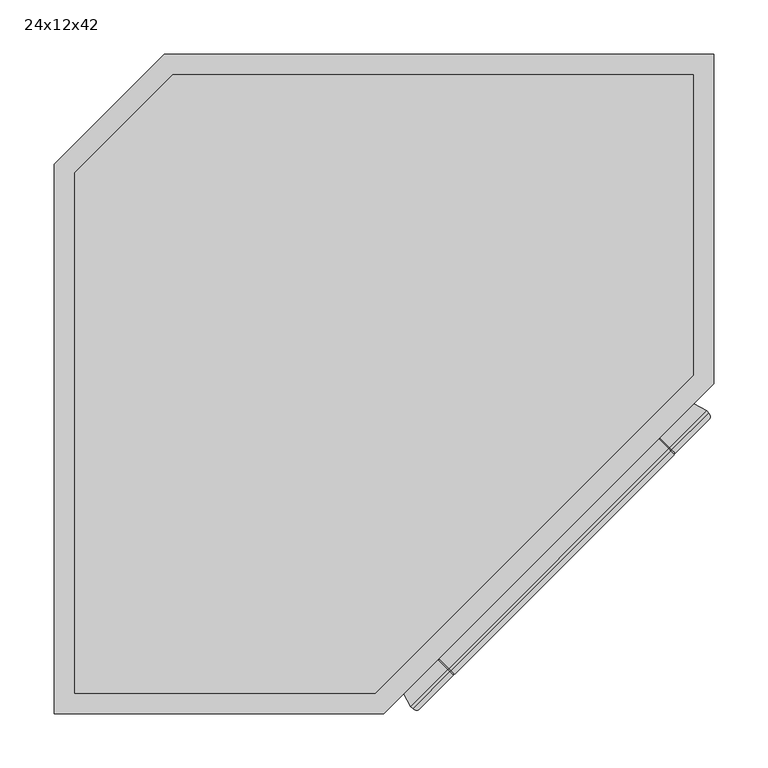
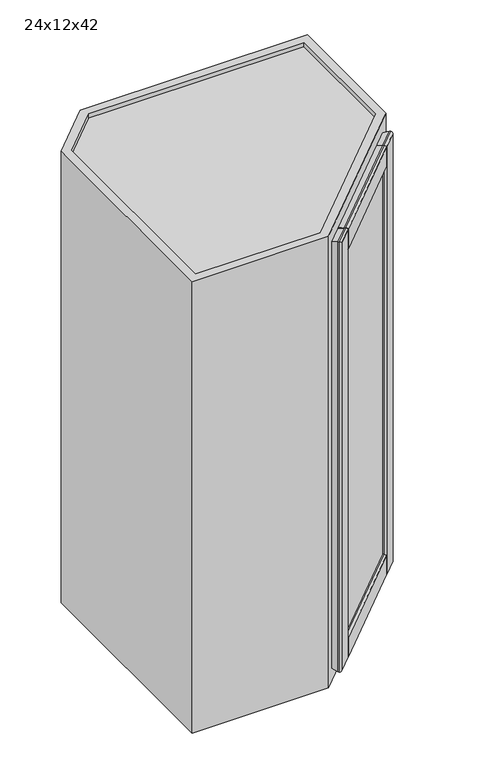
"""IFC4 building model written with IfcOpenShell, lengths in millimetres: furniture geometry, Cabinet-Wall-Merillat-Angle_Single_Door-Marlin : 24x12x42."""

from ifc_helpers import new_model, si_unit, frame, origin, place, context, project, spatial, polyline, circle_curve, ellipse_curve, outline, extrude, faceted_brep, source, transform, mapped, element, save
from ifc_brep_helpers import plane_surface, cylinder_surface, advanced_brep


def furniture_24x12x42_852458e2(model_context):
    return source(origin(), model_context, "Body", "SolidModel", [
        advanced_brep(
        [(-277.8609132, -57.3881325, 2451.1), (-277.8609132, -57.3881325, 1435.1), (-272.5103122, -58.3596318, 1438.1964925), (-272.5103122, -58.3596318, 2448.0035075), (-279.818609, -55.4304366, 2451.1), (-279.818609, -55.4304366, 1435.1), (-286.5897222, -43.7022222, 2447.5948), (-286.5897222, -43.7022222, 1438.6052), (-254.9849038, -12.0974038, 2402.8988372), (-254.1619151, -12.3969472, 2402.5287055), (-249.5344535, -14.0812055, 2400.4475465), (-249.5344535, -14.0812055, 1485.7524535), (-254.1619151, -12.3969472, 1483.6712945), (-254.9849038, -12.0974038, 1483.3011628), (-248.9402505, -16.6549814, 2401.847316), (-248.9402505, -16.6549814, 1484.352684), (-258.8946123, -26.9630247, 2416.175), (-258.8946123, -26.9630247, 1470.025), (-255.4821149, -30.3755221, 2416.175), (-255.4821149, -30.3755221, 1470.025), (-245.1740716, -20.4211603, 2401.847316), (-245.1740716, -20.4211603, 1484.352684), (-242.6002957, -21.0153633, 2400.4475465), (-242.6002957, -21.0153633, 1485.7524535), (-240.9160374, -25.6428249, 2402.5287055), (-240.6188146, -26.4594378, 2402.8959698), (-240.616494, -26.4658136, 1483.3011628), (-240.9160374, -25.6428249, 1483.6712945), (-3.5528682, 210.5978122, 1438.1964925), (-35.420563, 178.7301174, 1438.1964925), (-38.5816131, 181.8911676, 1435.1), (-4.5243675, 215.9484132, 1435.1), (-243.7755166, -23.3027358, 1435.1), (-240.6144664, -26.463786, 1438.1964925), (-242.6529845, -22.1802038, 1435.1), (-39.7041452, 180.7686356, 1435.1), (-36.543095, 177.6075854, 1438.1964925), (-239.4919344, -25.341254, 1438.1964925), (-40.539309, 183.8488634, 1435.1), (-6.4820634, 217.906109, 1435.1), (-245.7332124, -21.34504, 1435.1), (-244.6106804, -20.222508, 1435.1), (-41.661841, 182.7263314, 1435.1), (-49.7889728, 193.0985272, 1438.6052), (-18.2102778, 224.6772222, 1438.6052), (-254.9828762, -12.0953762, 1438.6052), (-253.8603442, -10.9728442, 1438.6052), (-50.9115048, 191.9759952, 1438.6052), (-47.8312945, 187.6219535, 1485.7524535), (-49.5155528, 192.2494151, 1483.6712945), (-50.3502388, 191.4147292, 1483.6712945), (-50.9115048, 191.9759952, 1483.3011628), (-253.8603442, -10.9728442, 1483.3011628), (-253.2990782, -11.5341102, 1483.6712945), (-45.2575186, 187.0277505, 1484.352684), (-34.9494753, 196.9821123, 1470.025), (-31.5369779, 193.5696149, 1470.025), (-41.4913397, 183.2615716, 1484.352684), (-40.8971367, 180.6877957, 1485.7524535), (-240.0532004, -24.779988, 1483.6712945), (-239.4919344, -25.341254, 1483.3011628), (-36.543095, 177.6075854, 1483.3011628), (-37.104361, 178.1688514, 1483.6712945), (-36.2696751, 179.0035374, 1483.6712945), (-4.5243675, 215.9484132, 2451.1), (-3.5528682, 210.5978122, 2448.0035075), (-6.4820634, 217.906109, 2451.1), (-18.2102778, 224.6772222, 2447.5948), (-49.8150962, 193.0724038, 1483.3011628), (-47.8312945, 187.6219535, 2400.4475465), (-49.5155528, 192.2494151, 2402.5287055), (-49.8150962, 193.0724038, 2402.8988372), (-45.2575186, 187.0277505, 2401.847316), (-34.9494753, 196.9821123, 2416.175), (-31.5369779, 193.5696149, 2416.175), (-41.4913397, 183.2615716, 2401.847316), (-40.8971367, 180.6877957, 2400.4475465), (-35.4466864, 178.703994, 1483.3011628), (-35.4466864, 178.703994, 2402.8988372), (-36.2696751, 179.0035374, 2402.5287055), (-240.6144664, -26.463786, 2448.0035075), (-243.7755166, -23.3027358, 2451.1), (-38.5816131, 181.8911676, 2451.1), (-35.420563, 178.7301174, 2448.0035075), (-39.7041452, 180.7686356, 2451.1), (-242.6529845, -22.1802038, 2451.1), (-239.4919344, -25.341254, 2448.0035075), (-36.543095, 177.6075854, 2448.0035075), (-245.7332124, -21.34504, 2451.1), (-40.539309, 183.8488634, 2451.1), (-41.661841, 182.7263314, 2451.1), (-244.6106804, -20.222508, 2451.1), (-254.9828762, -12.0953762, 2447.5948), (-49.7889728, 193.0985272, 2447.5948), (-50.9115048, 191.9759952, 2447.5948), (-253.8603442, -10.9728442, 2447.5948), (-50.9115048, 191.9759952, 2402.8988372), (-253.8603442, -10.9728442, 2402.8988372), (-253.2990782, -11.5341102, 2402.5287055), (-50.3502388, 191.4147292, 2402.5287055), (-37.104361, 178.1688514, 2402.5287055), (-36.543095, 177.6075854, 2402.8988372), (-239.4919344, -25.341254, 2402.8988372), (-240.0532004, -24.779988, 2402.5287055), (-37.104361, 178.1688514, 2447.8526052), (-39.7041452, 180.7686356, 2450.30625), (-41.5879457, 182.6524361, 2450.30625), (-50.3502388, 191.4147292, 2446.9857412), (-49.2277068, 192.5372612, 2402.5287055), (-49.2277068, 192.5372612, 2446.9857412), (-40.4654137, 183.7749682, 2450.30625), (-38.5816131, 181.8911676, 2450.30625), (-35.981829, 179.2913834, 2447.8526052), (-35.981829, 179.2913834, 2402.5287055), (-241.1757324, -25.90252, 2402.5287055), (-241.1757324, -25.90252, 2447.8526052), (-243.7755166, -23.3027358, 2450.30625), (-245.6593171, -21.4189353, 2450.30625), (-254.4216102, -12.6566422, 2446.9857412), (-254.4216102, -12.6566422, 2402.5287055), (-253.2990782, -11.5341102, 2446.9857412), (-244.5367851, -20.2964033, 2450.30625), (-242.6529845, -22.1802038, 2450.30625), (-240.0532004, -24.779988, 2447.8526052), (-254.4216102, -12.6566422, 1483.6712945), (-254.4216102, -12.6566422, 1439.2142588), (-245.6593171, -21.4189353, 1435.89375), (-243.7755166, -23.3027358, 1435.89375), (-241.1757324, -25.90252, 1438.3473948), (-241.1757324, -25.90252, 1483.6712945), (-240.0532004, -24.779988, 1438.3473948), (-242.6529845, -22.1802038, 1435.89375), (-244.5367851, -20.2964033, 1435.89375), (-253.2990782, -11.5341102, 1439.2142588), (-50.3502388, 191.4147292, 1439.2142588), (-41.5879457, 182.6524361, 1435.89375), (-39.7041452, 180.7686356, 1435.89375), (-37.104361, 178.1688514, 1438.3473948), (-35.981829, 179.2913834, 1483.6712945), (-35.981829, 179.2913834, 1438.3473948), (-38.5816131, 181.8911676, 1435.89375), (-40.4654137, 183.7749682, 1435.89375), (-49.2277068, 192.5372612, 1439.2142588), (-49.2277068, 192.5372612, 1483.6712945)],
        [
            (0, 1),
            (1, 2, ellipse_curve(frame((-274.4843369, -54.0115562, 1439.8752), z_axis=(-0.5000000000000054, -0.4999999999999945, 0.7071067811865475), x_axis=(0.5000000000000053, 0.4999999999999944, 0.7071067811865476)), 6.7531526, 4.7752)),
            (2, 3),
            (3, 0, ellipse_curve(frame((-274.4843369, -54.0115562, 2446.3248), z_axis=(-0.5000000000000054, -0.4999999999999945, -0.7071067811865475), x_axis=(-0.5000000000000053, -0.4999999999999944, 0.7071067811865476)), 6.7531526, 4.7752)),
            (0, 4),
            (4, 5),
            (5, 1),
            (4, 6),
            (6, 7),
            (7, 5),
            (8, 9),
            (9, 10),
            (10, 11),
            (11, 12),
            (12, 13),
            (13, 8),
            (10, 14, ellipse_curve(frame((-250.0730668, -15.5610334, 2401.8748), z_axis=(-0.5000000000000054, -0.4999999999999945, -0.7071067811865475), x_axis=(-0.5000000000000053, -0.4999999999999944, 0.7071067811865476)), 2.2271035, 1.5748)),
            (14, 15),
            (15, 11, ellipse_curve(frame((-250.0730668, -15.5610334, 1484.3252), z_axis=(-0.5000000000000054, -0.4999999999999945, 0.7071067811865475), x_axis=(0.5000000000000053, 0.4999999999999944, 0.7071067811865476)), 2.2271035, 1.5748)),
            (14, 16),
            (16, 17),
            (17, 15),
            (16, 18),
            (18, 19),
            (19, 17),
            (18, 20),
            (20, 21),
            (21, 19),
            (20, 22, ellipse_curve(frame((-244.0801236, -21.5539766, 2401.8748), z_axis=(-0.5000000000000054, -0.4999999999999945, -0.7071067811865475), x_axis=(-0.5000000000000053, -0.4999999999999944, 0.7071067811865476)), 2.2271035, 1.5748)),
            (22, 23),
            (23, 21, ellipse_curve(frame((-244.0801236, -21.5539766, 1484.3252), z_axis=(-0.5000000000000054, -0.4999999999999945, 0.7071067811865475), x_axis=(0.5000000000000053, 0.4999999999999944, 0.7071067811865476)), 2.2271035, 1.5748)),
            (22, 24),
            (24, 25),
            (25, 26),
            (26, 27),
            (27, 23),
            (28, 29),
            (29, 30, circle_curve(frame((-38.5816131, 181.8911676, 1439.8752), z_axis=(0.7071067811865552, 0.7071067811865398, 0.0), x_axis=(-0.7071067811865398, 0.7071067811865552, 0.0)), 4.7752)),
            (30, 31),
            (31, 28, ellipse_curve(frame((-7.9009438, 212.5718369, 1439.8752), z_axis=(-0.5000000000000054, -0.4999999999999945, -0.7071067811865475), x_axis=(-0.5000000000000054, -0.49999999999999456, 0.7071067811865474)), 6.7531526, 4.7752)),
            (1, 32),
            (32, 33, circle_curve(frame((-243.7755166, -23.3027358, 1439.8752), z_axis=(-0.7071067811865552, -0.7071067811865398, 0.0), x_axis=(-0.7071067811865398, 0.7071067811865552, 0.0)), 4.7752)),
            (33, 2),
            (34, 35),
            (35, 36, circle_curve(frame((-39.7041452, 180.7686356, 1439.8752), z_axis=(-0.7071067811865552, -0.7071067811865398, 0.0), x_axis=(-0.7071067811865398, 0.7071067811865552, 0.0)), 4.7752)),
            (36, 37),
            (37, 34, circle_curve(frame((-242.6529845, -22.1802038, 1439.8752), z_axis=(0.7071067811865552, 0.7071067811865398, 0.0), x_axis=(-0.7071067811865398, 0.7071067811865552, 0.0)), 4.7752)),
            (30, 38),
            (38, 39),
            (39, 31),
            (5, 40),
            (40, 32),
            (41, 42),
            (42, 35),
            (34, 41),
            (38, 43),
            (43, 44),
            (44, 39),
            (7, 45),
            (45, 40),
            (46, 47),
            (47, 42),
            (41, 46),
            (48, 49),
            (49, 50),
            (50, 51),
            (51, 52),
            (52, 53),
            (53, 12),
            (11, 48),
            (15, 54),
            (54, 48, ellipse_curve(frame((-46.3514666, 188.1605668, 1484.3252), z_axis=(-0.5000000000000054, -0.4999999999999945, -0.7071067811865475), x_axis=(-0.5000000000000054, -0.49999999999999456, 0.7071067811865474)), 2.2271035, 1.5748)),
            (17, 55),
            (55, 54),
            (19, 56),
            (56, 55),
            (21, 57),
            (57, 56),
            (23, 58),
            (58, 57, ellipse_curve(frame((-40.3585234, 182.1676236, 1484.3252), z_axis=(-0.5000000000000054, -0.4999999999999945, -0.7071067811865475), x_axis=(-0.5000000000000054, -0.49999999999999456, 0.7071067811865474)), 2.2271035, 1.5748)),
            (27, 59),
            (59, 60),
            (60, 61),
            (61, 62),
            (62, 63),
            (63, 58),
            (31, 64),
            (64, 65, ellipse_curve(frame((-7.9009438, 212.5718369, 2446.3248), z_axis=(0.5000000000000054, 0.4999999999999945, -0.7071067811865475), x_axis=(-0.5000000000000053, -0.4999999999999944, -0.7071067811865476)), 6.7531526, 4.7752)),
            (65, 28),
            (39, 66),
            (66, 64),
            (44, 67),
            (67, 66),
            (68, 49),
            (48, 69),
            (69, 70),
            (70, 71),
            (71, 68),
            (54, 72),
            (72, 69, ellipse_curve(frame((-46.3514666, 188.1605668, 2401.8748), z_axis=(0.5000000000000054, 0.4999999999999945, -0.7071067811865475), x_axis=(-0.5000000000000053, -0.4999999999999944, -0.7071067811865476)), 2.2271035, 1.5748)),
            (55, 73),
            (73, 72),
            (56, 74),
            (74, 73),
            (57, 75),
            (75, 74),
            (58, 76),
            (76, 75, ellipse_curve(frame((-40.3585234, 182.1676236, 2401.8748), z_axis=(0.5000000000000054, 0.4999999999999945, -0.7071067811865475), x_axis=(-0.5000000000000053, -0.4999999999999944, -0.7071067811865476)), 2.2271035, 1.5748)),
            (63, 77),
            (77, 78),
            (78, 79),
            (79, 76),
            (3, 80),
            (80, 81, circle_curve(frame((-243.7755166, -23.3027358, 2446.3248), z_axis=(-0.7071067811865552, -0.7071067811865398, 0.0), x_axis=(-0.7071067811865398, 0.7071067811865552, 0.0)), 4.7752)),
            (81, 0),
            (64, 82),
            (82, 83, circle_curve(frame((-38.5816131, 181.8911676, 2446.3248), z_axis=(0.7071067811865552, 0.7071067811865398, 0.0), x_axis=(-0.7071067811865398, 0.7071067811865552, 0.0)), 4.7752)),
            (83, 65),
            (84, 85),
            (85, 86, circle_curve(frame((-242.6529845, -22.1802038, 2446.3248), z_axis=(0.7071067811865552, 0.7071067811865398, 0.0), x_axis=(-0.7071067811865398, 0.7071067811865552, 0.0)), 4.7752)),
            (86, 87),
            (87, 84, circle_curve(frame((-39.7041452, 180.7686356, 2446.3248), z_axis=(-0.7071067811865552, -0.7071067811865398, 0.0), x_axis=(-0.7071067811865398, 0.7071067811865552, 0.0)), 4.7752)),
            (81, 88),
            (88, 4),
            (66, 89),
            (89, 82),
            (90, 91),
            (91, 85),
            (84, 90),
            (88, 92),
            (92, 6),
            (67, 93),
            (93, 89),
            (94, 95),
            (95, 91),
            (90, 94),
            (51, 47),
            (46, 52),
            (92, 8),
            (13, 45),
            (43, 68),
            (71, 93),
            (96, 97),
            (97, 95),
            (94, 96),
            (9, 98),
            (98, 97),
            (96, 99),
            (99, 70),
            (69, 10),
            (72, 14),
            (73, 16),
            (74, 18),
            (75, 20),
            (76, 22),
            (79, 100),
            (100, 101),
            (101, 102),
            (102, 103),
            (103, 24),
            (33, 26),
            (25, 80),
            (36, 61),
            (60, 37),
            (83, 78),
            (77, 29),
            (86, 102),
            (101, 87),
            (100, 104),
            (104, 105, circle_curve(frame((-39.7041452, 180.7686356, 2446.3248), z_axis=(-0.7071067811865624, -0.7071067811865326, 0.0), x_axis=(0.0, 0.0, 1.0)), 3.98145)),
            (105, 106),
            (106, 107),
            (107, 99),
            (71, 108),
            (108, 109),
            (109, 110),
            (110, 111),
            (111, 112, circle_curve(frame((-38.5816131, 181.8911676, 2446.3248), z_axis=(0.7071067811865624, 0.7071067811865326, 0.0), x_axis=(0.0, 0.0, 1.0)), 3.98145)),
            (112, 113),
            (113, 78),
            (113, 79),
            (112, 104),
            (111, 105),
            (110, 106),
            (109, 107),
            (108, 70),
            (25, 114),
            (114, 115),
            (115, 116, circle_curve(frame((-243.7755166, -23.3027358, 2446.3248), z_axis=(-0.7071067811865624, -0.7071067811865326, 0.0), x_axis=(0.0, 0.0, 1.0)), 3.98145)),
            (116, 117),
            (117, 118),
            (118, 119),
            (119, 8),
            (98, 120),
            (120, 121),
            (121, 122),
            (122, 123, circle_curve(frame((-242.6529845, -22.1802038, 2446.3248), z_axis=(0.7071067811865624, 0.7071067811865326, 0.0), x_axis=(0.0, 0.0, 1.0)), 3.98145)),
            (123, 103),
            (24, 114),
            (123, 115),
            (122, 116),
            (121, 117),
            (120, 118),
            (9, 119),
            (13, 124),
            (124, 125),
            (125, 126),
            (126, 127),
            (127, 128, circle_curve(frame((-243.7755166, -23.3027358, 1439.8752), z_axis=(-0.7071067811865624, -0.7071067811865326, 0.0), x_axis=(0.0, 0.0, 1.0)), 3.98145)),
            (128, 129),
            (129, 26),
            (59, 130),
            (130, 131, circle_curve(frame((-242.6529845, -22.1802038, 1439.8752), z_axis=(0.7071067811865624, 0.7071067811865326, 0.0), x_axis=(0.0, 0.0, 1.0)), 3.98145)),
            (131, 132),
            (132, 133),
            (133, 53),
            (12, 124),
            (133, 125),
            (132, 126),
            (131, 127),
            (130, 128),
            (27, 129),
            (50, 134),
            (134, 135),
            (135, 136),
            (136, 137, circle_curve(frame((-39.7041452, 180.7686356, 1439.8752), z_axis=(-0.7071067811865624, -0.7071067811865326, 0.0), x_axis=(0.0, 0.0, 1.0)), 3.98145)),
            (137, 62),
            (138, 139),
            (139, 140, circle_curve(frame((-38.5816131, 181.8911676, 1439.8752), z_axis=(0.7071067811865624, 0.7071067811865326, 0.0), x_axis=(0.0, 0.0, 1.0)), 3.98145)),
            (140, 141),
            (141, 142),
            (142, 143),
            (143, 68),
            (77, 138),
            (63, 138),
            (143, 49),
            (142, 134),
            (141, 135),
            (140, 136),
            (139, 137),
        ],
        [
            cylinder_surface(frame((-274.4843369, -54.0115562, 2451.1), z_axis=(0.0, 0.0, 1.0), x_axis=(-0.7071067811865386, 0.7071067811865565, 0.0)), 4.7752),
            plane_surface(frame((-277.8609132, -57.3881325, 2451.1), z_axis=(-0.7071067811865565, -0.7071067811865386, 0.0), x_axis=(0.0, 0.0, -1.0))),
            plane_surface(frame((-279.818609, -55.4304366, 2451.1), z_axis=(-0.8660309890157614, -0.4999903259707954, 0.0), x_axis=(0.0, 0.0, -1.0))),
            plane_surface(frame((-254.9849038, -12.0974038, 2402.8988372), z_axis=(0.3420201433255897, 0.9396926207859373, 0.0), x_axis=(0.0, 0.0, -1.0))),
            cylinder_surface(frame((-250.0730668, -15.5610334, 2451.1), z_axis=(0.0, 0.0, 1.0000000000000002), x_axis=(0.7193398003386506, -0.6946583704589979, 0.0)), 1.5748),
            plane_surface(frame((-248.9402505, -16.6549814, 2401.847316), z_axis=(0.7193398003386704, -0.6946583704589774, 0.0), x_axis=(0.0, 0.0, -1.0))),
            plane_surface(frame((-258.8946123, -26.9630247, 2416.175), z_axis=(0.7071067811865565, 0.7071067811865386, 0.0), x_axis=(0.0, 0.0, -1.0))),
            plane_surface(frame((-255.4821149, -30.3755221, 2416.175), z_axis=(-0.6946583704589931, 0.7193398003386553, 0.0), x_axis=(0.0, 0.0, -1.0))),
            cylinder_surface(frame((-244.0801236, -21.5539766, 2451.1), z_axis=(0.0, 0.0, 1.0000000000000002), x_axis=(0.9396926207858454, 0.3420201433258422, 0.0)), 1.5748),
            plane_surface(frame((-242.6002957, -21.0153633, 2400.4475465), z_axis=(0.9396926207859256, 0.3420201433256214, 0.0), x_axis=(0.0, 0.0, -1.0))),
            cylinder_surface(frame((-277.8609132, -57.3881325, 1439.8752), z_axis=(-0.7071067811865552, -0.7071067811865398, 0.0), x_axis=(-0.7071067811865398, 0.7071067811865552, 0.0)), 4.7752),
            plane_surface(frame((-277.8609132, -57.3881325, 1435.1), z_axis=(0.0, 0.0, -1.0), x_axis=(0.7071067811865552, 0.7071067811865398, 0.0))),
            plane_surface(frame((-279.818609, -55.4304366, 1435.1), z_axis=(-0.18302033152247357, 0.18302033152247757, -0.9659229350723619), x_axis=(0.7071067811865552, 0.7071067811865398, 0.0))),
            plane_surface(frame((-254.9849038, -12.0974038, 1483.3011628), z_axis=(-0.2988362387301775, 0.298836238730184, 0.9063077870366099), x_axis=(0.7071067811865552, 0.7071067811865398, 0.0))),
            cylinder_surface(frame((-284.8805396, -50.3685061, 1484.3252), z_axis=(-0.7071067811865553, -0.7071067811865399, 0.0), x_axis=(0.7069990853988164, -0.7069990853988318, 0.01745240643729364)), 1.5748),
            plane_surface(frame((-248.9402505, -16.6549814, 1484.352684), z_axis=(0.7069990853988161, -0.7069990853988315, 0.017452406437322144), x_axis=(0.7071067811865552, 0.7071067811865398, 0.0))),
            plane_surface(frame((-258.8946123, -26.9630247, 1470.025), z_axis=(0.0, 0.0, 1.0), x_axis=(0.7071067811865552, 0.7071067811865398, 0.0))),
            plane_surface(frame((-255.4821149, -30.3755221, 1470.025), z_axis=(-0.7069990853988166, 0.706999085398832, 0.01745240643727848), x_axis=(0.7071067811865552, 0.7071067811865398, 0.0))),
            cylinder_surface(frame((-278.8875963, -56.3614494, 1484.3252), z_axis=(-0.7071067811865553, -0.7071067811865399, 0.0), x_axis=(0.2988362387299914, -0.29883623872999787, 0.9063077870367326)), 1.5748),
            plane_surface(frame((-242.6002957, -21.0153633, 1485.7524535), z_axis=(0.29883623873014187, -0.29883623873014836, 0.9063077870366333), x_axis=(0.7071067811865552, 0.7071067811865398, 0.0))),
            cylinder_surface(frame((-7.9009438, 212.5718369, 1435.1), z_axis=(0.0, 0.0, -1.0), x_axis=(-0.707106781186541, 0.707106781186554, 0.0)), 4.7752),
            plane_surface(frame((-4.5243675, 215.9484132, 1435.1), z_axis=(0.707106781186554, 0.707106781186541, 0.0), x_axis=(0.0, 0.0, 1.0))),
            plane_surface(frame((-6.4820634, 217.906109, 1435.1), z_axis=(0.4999903259708143, 0.8660309890157505, 0.0), x_axis=(0.0, 0.0, 1.0))),
            plane_surface(frame((-49.8150962, 193.0724038, 1483.3011628), z_axis=(-0.9396926207859447, -0.34202014332556924, 0.0), x_axis=(0.0, 0.0, 1.0))),
            cylinder_surface(frame((-46.3514666, 188.1605668, 1435.1), z_axis=(0.0, 0.0, -1.0000000000000002), x_axis=(0.6946583704589822, -0.7193398003386657, 0.0)), 1.5748),
            plane_surface(frame((-45.2575186, 187.0277505, 1484.352684), z_axis=(0.6946583704589617, -0.7193398003386856, 0.0), x_axis=(0.0, 0.0, 1.0))),
            plane_surface(frame((-34.9494753, 196.9821123, 1470.025), z_axis=(-0.707106781186554, -0.707106781186541, 0.0), x_axis=(0.0, 0.0, 1.0))),
            plane_surface(frame((-31.5369779, 193.5696149, 1470.025), z_axis=(-0.7193398003386401, 0.6946583704590088, 0.0), x_axis=(0.0, 0.0, 1.0))),
            cylinder_surface(frame((-40.3585234, 182.1676236, 1435.1), z_axis=(0.0, 0.0, -1.0000000000000002), x_axis=(-0.34202014332586267, -0.9396926207858379, 0.0)), 1.5748),
            plane_surface(frame((-40.8971367, 180.6877957, 1485.7524535), z_axis=(-0.3420201433256419, -0.9396926207859182, 0.0), x_axis=(0.0, 0.0, 1.0))),
            cylinder_surface(frame((-4.5243675, 215.9484132, 2446.3248), z_axis=(0.7071067811865552, 0.7071067811865398, 0.0), x_axis=(-0.7071067811865398, 0.7071067811865552, 0.0)), 4.7752),
            plane_surface(frame((-4.5243675, 215.9484132, 2451.1), z_axis=(0.0, 0.0, 1.0), x_axis=(-0.7071067811865552, -0.7071067811865398, 0.0))),
            plane_surface(frame((-6.4820634, 217.906109, 2451.1), z_axis=(-0.18302033152247357, 0.18302033152247757, 0.9659229350723619), x_axis=(-0.7071067811865552, -0.7071067811865398, 0.0))),
            plane_surface(frame((-18.2102778, 224.6772222, 2447.5948), z_axis=(-0.7071067811865398, 0.7071067811865552, 0.0), x_axis=(-0.7071067811865552, -0.7071067811865398, 0.0))),
            plane_surface(frame((-49.8150962, 193.0724038, 2402.8988372), z_axis=(-0.2988362387301775, 0.298836238730184, -0.9063077870366099), x_axis=(-0.7071067811865552, -0.7071067811865398, 0.0))),
            cylinder_surface(frame((-11.5439939, 222.9680396, 2401.8748), z_axis=(0.7071067811865553, 0.7071067811865399, 0.0), x_axis=(0.7069990853988164, -0.7069990853988318, -0.01745240643729364)), 1.5748),
            plane_surface(frame((-45.2575186, 187.0277505, 2401.847316), z_axis=(0.7069990853988161, -0.7069990853988315, -0.017452406437322144), x_axis=(-0.7071067811865552, -0.7071067811865398, 0.0))),
            plane_surface(frame((-34.9494753, 196.9821123, 2416.175), z_axis=(0.0, 0.0, -1.0), x_axis=(-0.7071067811865552, -0.7071067811865398, 0.0))),
            plane_surface(frame((-31.5369779, 193.5696149, 2416.175), z_axis=(-0.7069990853988166, 0.706999085398832, -0.01745240643727848), x_axis=(-0.7071067811865552, -0.7071067811865398, 0.0))),
            cylinder_surface(frame((-5.5510506, 216.9750963, 2401.8748), z_axis=(0.7071067811865553, 0.7071067811865399, 0.0), x_axis=(0.2988362387299914, -0.29883623872999787, -0.9063077870367326)), 1.5748),
            plane_surface(frame((-40.8971367, 180.6877957, 2400.4475465), z_axis=(0.29883623873014187, -0.29883623873014836, -0.9063077870366333), x_axis=(-0.7071067811865552, -0.7071067811865398, 0.0))),
            plane_surface(frame((-35.4466864, 178.703994, 2402.8988372), z_axis=(0.7071067811865398, -0.7071067811865552, 0.0), x_axis=(-0.7071067811865552, -0.7071067811865398, 0.0))),
            plane_surface(frame((-36.543095, 177.6075854, 2402.8988372), z_axis=(0.7071067811865626, 0.7071067811865326, 0.0), x_axis=(-0.6408563820557467, 0.6408563820557738, -0.4226182617407854))),
            plane_surface(frame((-35.420563, 178.7301174, 2402.8988372), z_axis=(-0.7071067811865626, -0.7071067811865326, 0.0), x_axis=(0.6408563820557467, -0.6408563820557738, 0.4226182617407854))),
            plane_surface(frame((-36.543095, 177.6075854, 2402.8988372), z_axis=(-0.2988362387301741, 0.29883623873018705, 0.9063077870366099), x_axis=(0.7071067811865628, 0.7071067811865323, 0.0))),
            plane_surface(frame((-37.104361, 178.1688514, 2402.5287055), z_axis=(0.7071067811865323, -0.7071067811865628, 0.0), x_axis=(0.7071067811865628, 0.7071067811865323, 0.0))),
            cylinder_surface(frame((-38.5816131, 181.8911676, 2446.3248), z_axis=(0.7071067811865624, 0.7071067811865326, 0.0), x_axis=(0.0, 0.0, 1.0)), 3.98145),
            plane_surface(frame((-39.7041452, 180.7686356, 2450.30625), z_axis=(0.0, 0.0, 1.0), x_axis=(0.7071067811865628, 0.7071067811865323, 0.0))),
            plane_surface(frame((-41.5879457, 182.6524361, 2450.30625), z_axis=(-0.18302033152251368, 0.18302033152252156, 0.9659229350723461), x_axis=(0.7071067811865628, 0.7071067811865323, 0.0))),
            plane_surface(frame((-50.3502388, 191.4147292, 2446.9857412), z_axis=(-0.7071067811865323, 0.7071067811865628, 0.0), x_axis=(0.7071067811865628, 0.7071067811865323, 0.0))),
            plane_surface(frame((-50.3502388, 191.4147292, 2402.5287055), z_axis=(0.2988362387301922, -0.29883623873020515, 0.906307787036598), x_axis=(0.7071067811865628, 0.7071067811865323, 0.0))),
            plane_surface(frame((-240.6144664, -26.463786, 2402.8988372), z_axis=(0.7071067811865626, 0.7071067811865326, 0.0), x_axis=(-0.6408563820557467, 0.6408563820557738, -0.4226182617407854))),
            plane_surface(frame((-239.4919344, -25.341254, 2402.8988372), z_axis=(-0.7071067811865626, -0.7071067811865326, 0.0), x_axis=(0.6408563820557467, -0.6408563820557738, 0.4226182617407854))),
            plane_surface(frame((-240.6144664, -26.463786, 2402.8988372), z_axis=(-0.2988362387301741, 0.29883623873018705, 0.9063077870366099), x_axis=(0.7071067811865628, 0.7071067811865323, 0.0))),
            plane_surface(frame((-241.1757324, -25.90252, 2402.5287055), z_axis=(0.7071067811865323, -0.7071067811865628, 0.0), x_axis=(0.7071067811865628, 0.7071067811865323, 0.0))),
            cylinder_surface(frame((-242.6529845, -22.1802038, 2446.3248), z_axis=(0.7071067811865624, 0.7071067811865326, 0.0), x_axis=(0.0, 0.0, 1.0)), 3.98145),
            plane_surface(frame((-243.7755166, -23.3027358, 2450.30625), z_axis=(0.0, 0.0, 1.0), x_axis=(0.7071067811865628, 0.7071067811865323, 0.0))),
            plane_surface(frame((-245.6593171, -21.4189353, 2450.30625), z_axis=(-0.18302033152251543, 0.18302033152252334, 0.9659229350723453), x_axis=(0.7071067811865628, 0.7071067811865323, 0.0))),
            plane_surface(frame((-254.4216102, -12.6566422, 2446.9857412), z_axis=(-0.7071067811865341, 0.7071067811865609, 0.0), x_axis=(0.7071067811865609, 0.7071067811865341, 0.0))),
            plane_surface(frame((-254.4216102, -12.6566422, 2402.5287055), z_axis=(0.29883623873019366, -0.298836238730205, 0.9063077870365974), x_axis=(0.7071067811865609, 0.7071067811865341, 0.0))),
            plane_surface(frame((-243.7755166, -23.3027358, 1444.6504), z_axis=(0.7071067811865624, 0.7071067811865326, 0.0), x_axis=(0.7071067811865326, -0.7071067811865624, 0.0))),
            plane_surface(frame((-242.6529845, -22.1802038, 1444.6504), z_axis=(-0.7071067811865624, -0.7071067811865326, 0.0), x_axis=(-0.7071067811865326, 0.7071067811865624, 0.0))),
            plane_surface(frame((-254.9828762, -12.0953762, 1483.3011628), z_axis=(0.2988362387301802, -0.2988362387301931, -0.906307787036606), x_axis=(0.7071067811865628, 0.7071067811865323, 0.0))),
            plane_surface(frame((-254.4216102, -12.6566422, 1483.6712945), z_axis=(-0.7071067811865323, 0.7071067811865628, 0.0), x_axis=(0.7071067811865628, 0.7071067811865323, 0.0))),
            plane_surface(frame((-254.4216102, -12.6566422, 1439.2142588), z_axis=(-0.18302033152271613, 0.18302033152272404, -0.9659229350722693), x_axis=(0.7071067811865628, 0.7071067811865323, 0.0))),
            plane_surface(frame((-245.6593171, -21.4189353, 1435.89375), z_axis=(0.0, 0.0, -1.0), x_axis=(0.7071067811865628, 0.7071067811865323, 0.0))),
            cylinder_surface(frame((-242.6529845, -22.1802038, 1439.8752), z_axis=(0.7071067811865624, 0.7071067811865326, 0.0), x_axis=(0.0, 0.0, 1.0)), 3.98145),
            plane_surface(frame((-241.1757324, -25.90252, 1438.3473948), z_axis=(0.7071067811865323, -0.7071067811865628, 0.0), x_axis=(0.7071067811865628, 0.7071067811865323, 0.0))),
            plane_surface(frame((-241.1757324, -25.90252, 1483.6712945), z_axis=(-0.2988362387301788, 0.2988362387301917, -0.9063077870366069), x_axis=(0.7071067811865628, 0.7071067811865323, 0.0))),
            plane_surface(frame((-37.104361, 178.1688514, 1483.6712945), z_axis=(0.7071067811865626, 0.7071067811865327, 0.0), x_axis=(0.6408563820557602, -0.6408563820557873, -0.42261826174074446))),
            plane_surface(frame((-35.981829, 179.2913834, 1483.6712945), z_axis=(-0.7071067811865626, -0.7071067811865327, 0.0), x_axis=(-0.6408563820557602, 0.6408563820557873, 0.42261826174074446))),
            plane_surface(frame((-37.104361, 178.1688514, 1483.6712945), z_axis=(-0.2988362387301452, 0.29883623873015813, -0.9063077870366291), x_axis=(0.7071067811865628, 0.7071067811865323, 0.0))),
            plane_surface(frame((-50.9115048, 191.9759952, 1483.3011628), z_axis=(0.2988362387301802, -0.2988362387301931, -0.906307787036606), x_axis=(0.7071067811865628, 0.7071067811865323, 0.0))),
            plane_surface(frame((-50.3502388, 191.4147292, 1483.6712945), z_axis=(-0.7071067811865323, 0.7071067811865628, 0.0), x_axis=(0.7071067811865628, 0.7071067811865323, 0.0))),
            plane_surface(frame((-50.3502388, 191.4147292, 1439.2142588), z_axis=(-0.18302033152271618, 0.18302033152272407, -0.9659229350722693), x_axis=(0.7071067811865628, 0.7071067811865323, 0.0))),
            plane_surface(frame((-41.5879457, 182.6524361, 1435.89375), z_axis=(0.0, 0.0, -1.0), x_axis=(0.7071067811865628, 0.7071067811865323, 0.0))),
            cylinder_surface(frame((-38.5816131, 181.8911676, 1439.8752), z_axis=(0.7071067811865624, 0.7071067811865326, 0.0), x_axis=(0.0, 0.0, 1.0)), 3.98145),
            plane_surface(frame((-37.104361, 178.1688514, 1438.3473948), z_axis=(0.7071067811865323, -0.7071067811865628, 0.0), x_axis=(0.7071067811865628, 0.7071067811865323, 0.0))),
        ],
        [
            (0, [[1, 2, 3, 4]]),
            (1, [[5, 6, 7, -1]]),
            (2, [[8, 9, 10, -6]]),
            (3, [[11, 12, 13, 14, 15, 16]]),
            (4, [[17, 18, 19, -13]]),
            (5, [[20, 21, 22, -18]]),
            (6, [[23, 24, 25, -21]]),
            (7, [[26, 27, 28, -24]]),
            (8, [[29, 30, 31, -27]]),
            (9, [[32, 33, 34, 35, 36, -30]]),
            (10, [[37, 38, 39, 40]]),
            (10, [[41, 42, 43, -2]]),
            (10, [[44, 45, 46, 47]]),
            (11, [[-39, 48, 49, 50]]),
            (11, [[51, 52, -41, -7]]),
            (11, [[53, 54, -44, 55]]),
            (12, [[-49, 56, 57, 58]]),
            (12, [[59, 60, -51, -10]]),
            (12, [[61, 62, -53, 63]]),
            (13, [[64, 65, 66, 67, 68, 69, -14, 70]]),
            (14, [[71, 72, -70, -19]]),
            (15, [[73, 74, -71, -22]]),
            (16, [[75, 76, -73, -25]]),
            (17, [[77, 78, -75, -28]]),
            (18, [[79, 80, -77, -31]]),
            (19, [[-36, 81, 82, 83, 84, 85, 86, -79]]),
            (20, [[87, 88, 89, -40]]),
            (21, [[90, 91, -87, -50]]),
            (22, [[92, 93, -90, -58]]),
            (23, [[94, -64, 95, 96, 97, 98]]),
            (24, [[99, 100, -95, -72]]),
            (25, [[101, 102, -99, -74]]),
            (26, [[103, 104, -101, -76]]),
            (27, [[105, 106, -103, -78]]),
            (28, [[107, 108, -105, -80]]),
            (29, [[-86, 109, 110, 111, 112, -107]]),
            (30, [[113, 114, 115, -4]]),
            (30, [[116, 117, 118, -88]]),
            (30, [[119, 120, 121, 122]]),
            (31, [[-115, 123, 124, -5]]),
            (31, [[125, 126, -116, -91]]),
            (31, [[127, 128, -119, 129]]),
            (32, [[-124, 130, 131, -8]]),
            (32, [[132, 133, -125, -93]]),
            (32, [[134, 135, -127, 136]]),
            (33, [[-67, 137, -61, 138]]),
            (33, [[-131, 139, -16, 140, -59, -9]]),
            (33, [[-57, 141, -98, 142, -132, -92]]),
            (33, [[143, 144, -134, 145]]),
            (34, [[-12, 146, 147, -143, 148, 149, -96, 150]]),
            (35, [[-150, -100, 151, -17]]),
            (36, [[-151, -102, 152, -20]]),
            (37, [[-152, -104, 153, -23]]),
            (38, [[-153, -106, 154, -26]]),
            (39, [[-154, -108, 155, -29]]),
            (40, [[-112, 156, 157, 158, 159, 160, -32, -155]]),
            (41, [[-43, 161, -34, 162, -113, -3]]),
            (41, [[-46, 163, -83, 164]]),
            (41, [[-118, 165, -110, 166, -37, -89]]),
            (41, [[-121, 167, -158, 168]]),
            (42, [[-148, -145, -136, -129, -122, -168, -157, 169, 170, 171, 172, 173]]),
            (43, [[-165, -117, -126, -133, -142, 174, 175, 176, 177, 178, 179, 180]]),
            (44, [[181, -111, -180]]),
            (45, [[-156, -181, -179, 182, -169]]),
            (46, [[-182, -178, 183, -170]]),
            (47, [[-183, -177, 184, -171]]),
            (48, [[-184, -176, 185, -172]]),
            (49, [[-185, -175, 186, -149, -173]]),
            (50, [[-97, -186, -174]]),
            (51, [[-139, -130, -123, -114, -162, 187, 188, 189, 190, 191, 192, 193]]),
            (52, [[-159, -167, -120, -128, -135, -144, -147, 194, 195, 196, 197, 198]]),
            (53, [[-33, 199, -187]]),
            (54, [[-199, -160, -198, 200, -188]]),
            (55, [[-200, -197, 201, -189]]),
            (56, [[-201, -196, 202, -190]]),
            (57, [[-202, -195, 203, -191]]),
            (58, [[-203, -194, -146, 204, -192]]),
            (59, [[-204, -11, -193]]),
            (60, [[-161, -42, -52, -60, -140, 205, 206, 207, 208, 209, 210, 211]]),
            (61, [[-68, -138, -63, -55, -47, -164, -82, 212, 213, 214, 215, 216]]),
            (62, [[-15, 217, -205]]),
            (63, [[-217, -69, -216, 218, -206]]),
            (64, [[-218, -215, 219, -207]]),
            (65, [[-219, -214, 220, -208]]),
            (66, [[-220, -213, 221, -209]]),
            (67, [[-221, -212, -81, 222, -210]]),
            (68, [[-222, -35, -211]]),
            (69, [[-84, -163, -45, -54, -62, -137, -66, 223, 224, 225, 226, 227]]),
            (70, [[228, 229, 230, 231, 232, 233, -141, -56, -48, -38, -166, 234]]),
            (71, [[-109, 235, -234]]),
            (72, [[236, -94, -233]]),
            (73, [[-65, -236, -232, 237, -223]]),
            (74, [[-237, -231, 238, -224]]),
            (75, [[-238, -230, 239, -225]]),
            (76, [[-239, -229, 240, -226]]),
            (77, [[-240, -228, -235, -85, -227]]),
        ],
    ),
        extrude(outline(polyline([(-31.5369779, 193.5696149), (-255.4821149, -30.3755221), (-258.8946123, -26.9630247), (-34.9494753, 196.9821123), (-31.5369779, 193.5696149)])), frame((0.0, 0.0, 1470.025), z_axis=(0.0, 0.0, 1.0), x_axis=(1.0, 0.0, 0.0)), (0.0, 0.0, 1.0), 946.15),
        faceted_brep([(-296.0453842, -26.2171158, 2438.4), (-35.6953842, 234.1328842, 2438.4), (-22.225, 220.6625, 2438.4), (-282.575, -39.6875, 2438.4), (-35.6953842, 234.1328842, 1447.8), (-296.0453842, -26.2171158, 1447.8), (-282.575, -39.6875, 1447.8), (-22.225, 220.6625, 1447.8), (-609.6, -61.9125, 2476.5), (-304.8, -61.9125, 2476.5), (0.0, 242.8875, 2476.5), (0.0, 547.6875, 2476.5), (-508.0, 547.6875, 2476.5), (-609.6, 446.0875, 2476.5), (-19.05, 250.7782684, 2476.5), (-312.6907684, -42.8625, 2476.5), (-590.55, -42.8625, 2476.5), (-590.55, 438.1967316, 2476.5), (-500.1092316, 528.6375, 2476.5), (-19.05, 528.6375, 2476.5), (-609.6, -61.9125, 1409.7), (-609.6, 446.0875, 1409.7), (-508.0, 547.6875, 1409.7), (0.0, 547.6875, 1409.7), (0.0, 242.8875, 1409.7), (-304.8, -61.9125, 1409.7), (-19.05, 250.7782684, 1409.7), (-19.05, 528.6375, 1409.7), (-500.1092316, 528.6375, 1409.7), (-590.55, 438.1967316, 1409.7), (-590.55, -42.8625, 1409.7), (-312.6907684, -42.8625, 1409.7)], [[[0, 1, 2, 3]], [[4, 5, 6, 7]], [[1, 4, 7, 2]], [[3, 6, 5, 0]], [[8, 9, 10, 11, 12, 13], [14, 15, 16, 17, 18, 19]], [[20, 21, 22, 23, 24, 25], [26, 27, 28, 29, 30, 31]], [[13, 21, 20, 8]], [[12, 22, 21, 13]], [[11, 23, 22, 12]], [[10, 24, 23, 11]], [[9, 25, 24, 10], [2, 7, 6, 3]], [[8, 20, 25, 9]], [[19, 27, 26, 14]], [[18, 28, 27, 19]], [[17, 29, 28, 18]], [[16, 30, 29, 17]], [[15, 31, 30, 16]], [[14, 26, 31, 15], [0, 5, 4, 1]]]),
        extrude(outline(polyline([(-312.6907684, -42.8625), (-590.55, -42.8625), (-590.55, 438.1967316), (-500.1092316, 528.6375), (-19.05, 528.6375), (-19.05, 250.7782684), (-312.6907684, -42.8625)])), frame((0.0, 0.0, 2200.275), z_axis=(0.0, 0.0, 1.0), x_axis=(1.0, 0.0, 0.0)), (0.0, 0.0, 1.0), 19.05),
        extrude(outline(polyline([(-312.6907684, -42.8625), (-590.55, -42.8625), (-590.55, 438.1967316), (-500.1092316, 528.6375), (-19.05, 528.6375), (-19.05, 250.7782684), (-312.6907684, -42.8625)])), frame((0.0, 0.0, 1933.575), z_axis=(0.0, 0.0, 1.0), x_axis=(1.0, 0.0, 0.0)), (0.0, 0.0, 1.0), 19.05),
        extrude(outline(polyline([(-312.6907684, -42.8625), (-590.55, -42.8625), (-590.55, 438.1967316), (-500.1092316, 528.6375), (-19.05, 528.6375), (-19.05, 250.7782684), (-312.6907684, -42.8625)])), frame((0.0, 0.0, 1666.875), z_axis=(0.0, 0.0, 1.0), x_axis=(1.0, 0.0, 0.0)), (0.0, 0.0, 1.0), 19.05),
        extrude(outline(polyline([(-590.55, 438.1967316), (-500.1092316, 528.6375), (-19.05, 528.6375), (-19.05, 250.7782684), (-312.6907684, -42.8625), (-590.55, -42.8625), (-590.55, 438.1967316)])), frame((0.0, 0.0, 2447.925), z_axis=(0.0, 0.0, 1.0), x_axis=(1.0, 0.0, 0.0)), (0.0, 0.0, 1.0), 19.05),
        extrude(outline(polyline([(-312.6907684, -42.8625), (-590.55, -42.8625), (-590.55, 438.1967316), (-500.1092316, 528.6375), (-19.05, 528.6375), (-19.05, 250.7782684), (-312.6907684, -42.8625)])), frame((0.0, 0.0, 1419.225), z_axis=(0.0, 0.0, 1.0), x_axis=(1.0, 0.0, 0.0)), (0.0, 0.0, 1.0), 19.05),
    ])


if __name__ == "__main__":
    model = new_model("IFC4")
    model_context = context("Model", 3, world=origin())
    ifc_project = project(units=[si_unit("LENGTHUNIT", "METRE", prefix="MILLI")], contexts=[model_context])
    site = spatial("IfcSite", under=ifc_project)
    building = spatial("IfcBuilding", under=site)
    placement = place(None, origin())
    furniture_24x12x42_shape = furniture_24x12x42_852458e2(model_context)
    element("IfcFurniture", 1, ObjectType="Cabinet-Wall-Merillat-Angle_Single_Door-Marlin : 24x12x42", at=placement, inside=building, context=model_context, shape_type="MappedRepresentation", body=[
        mapped(furniture_24x12x42_shape, transform((0.0, 0.0, 0.0), x_axis=(1.0, 0.0, 0.0), y_axis=(0.0, 1.0, 0.0), z_axis=(0.0, 0.0, 1.0))),
    ])
    save(model, "model.ifc")

# Revit data of these elements
# Type "Cabinet-Wall-Merillat-Angle_Single_Door-Marlin : 24x12x42"
#   URL = "http://www.merillat.com/"
#   Product Page URL = "http://www.merillat.com/our-products/"
#   Product Line = "\"Express\""
#   Product Group = "Wall Cabinet"
#   Product Documentation Link = "http://merillatbusiness.com/wp-content/uploads/2014/07/Merillat_Classic_Catalog.pdf"
#   Model = "WA2442 R or L"
#   Manufacturer = "Merillat"
#   Glass Door Note = "Glass Cabinet doors are only available in specific sizes. Please refer to the catalog for this information before requesting a glass size"
#   Finish = "Wood"
#   Description = "Wall Angle Single Door Cabinet"
#   Construction Type = "Wall Angle Cabinet"
#   Cabinet Construction Note = "Requires 24  1/16 inches of wall space excluding dining room side cabinet door"
#   Assembly Code = "C1030410"
#   Width = 2' - 0"
#   Top of Cabinet = 8' - 0"
#   Spacing = 0' - 1"
#   Shelving Height = 0' - 10 1/2"
#   Height = 3' - 6"
#   Door Spacing = 0' - 1 3/4"
#   Depth = 1' - 0"
#   Cabinet Shell = 0' - 0 3/4"
#   Cabinet Door Width = 1' - 3 7/32"
#   Cabinet Door Height = 3' - 4"
#   COBie.Type = no
#   Solid Panel Door = no
#   Partial Overlay = yes
#   Number of Shelves = 3
#   Middle Shelf = yes
#   Glass Door = yes
#   Full Overlay = no
#   Elevation Swing Line = yes
#   Door Drawer Material = Wood - Merillat - Pecan(1)
#   Cabinet Material = Wood - Merillat - Pecan(1)
# Element 1 (IfcFurniture, "Cabinet-Wall-Merillat-Angle_Single_Door-Marlin : 24x12x42")
#   Materials on its faces: "Wood - Merillat - Pecan(1)"
# Materials
#   "Wood - Merillat - Pecan(1)": class "Wood", colour RGB 108 67 43, transparency 0, Cost = 0
